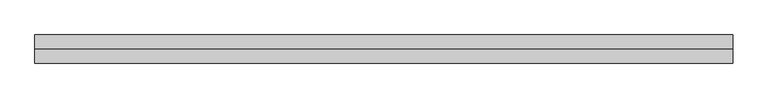
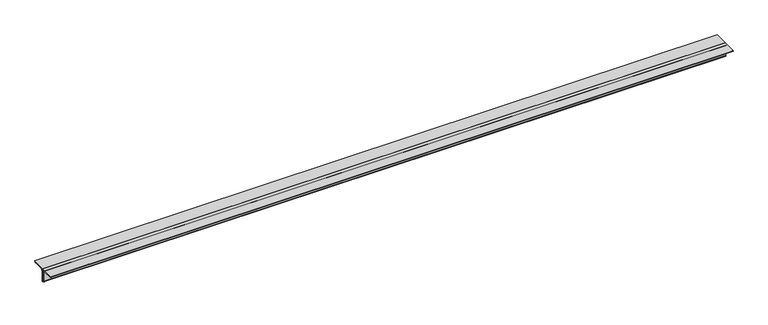
"""IFC4 building model written with IfcOpenShell, lengths in millimetres: member geometry, Steel Framing_2Ls_KS : H_SB_AR_S02_2Ls-100x100x10_VBR1."""

from ifc_helpers import new_model, si_unit, point, frame, frame_2d, origin, place, context, project, spatial, polyline, circle_curve, trimmed, segment, composite_curve, outline, extrude, source, transform, mapped, element, save


def member_093f2165(model_context):
    return source(origin(), model_context, "Body", "SweptSolid", [
        extrude(outline(composite_curve([segment(polyline([(0.0, 28.2), (100.0, 28.2)]), True, "CONTINUOUS"), segment(trimmed(circle_curve(frame_2d((90.0, 28.2)), 10.0), [point((100.0, 28.2))], [point((90.0, 18.2))], False, "CARTESIAN"), True, "CONTINUOUS"), segment(polyline([(90.0, 18.2), (20.0, 18.2)]), True, "CONTINUOUS"), segment(trimmed(circle_curve(frame_2d((20.0, 8.2)), 10.0), [point((20.0, 18.2))], [point((10.0, 8.2))], True, "CARTESIAN"), True, "CONTINUOUS"), segment(polyline([(10.0, 8.2), (10.0, -61.8)]), True, "CONTINUOUS"), segment(trimmed(circle_curve(frame_2d((0.0, -61.8)), 10.0), [point((10.0, -61.8))], [point((0.0, -71.8))], False, "CARTESIAN"), True, "CONTINUOUS"), segment(polyline([(0.0, -71.8), (0.0, 28.2)]), True, "CONTINUOUS")], self_intersect=False)), frame((-2479.1576866, 0.0, 0.0), z_axis=(1.0, 0.0, 0.0), x_axis=(0.0, 1.0, 0.0)), (0.0, 0.0, 1.0), 4958.3153733),
        extrude(outline(composite_curve([segment(polyline([(0.0, 28.2), (0.0, -71.8)]), True, "CONTINUOUS"), segment(trimmed(circle_curve(frame_2d((0.0, -61.8)), 10.0), [point((0.0, -71.8))], [point((-10.0, -61.8))], False, "CARTESIAN"), True, "CONTINUOUS"), segment(polyline([(-10.0, -61.8), (-10.0, 8.2)]), True, "CONTINUOUS"), segment(trimmed(circle_curve(frame_2d((-20.0, 8.2)), 10.0), [point((-10.0, 8.2))], [point((-20.0, 18.2))], True, "CARTESIAN"), True, "CONTINUOUS"), segment(polyline([(-20.0, 18.2), (-90.0, 18.2)]), True, "CONTINUOUS"), segment(trimmed(circle_curve(frame_2d((-90.0, 28.2)), 10.0), [point((-90.0, 18.2))], [point((-100.0, 28.2))], False, "CARTESIAN"), True, "CONTINUOUS"), segment(polyline([(-100.0, 28.2), (0.0, 28.2)]), True, "CONTINUOUS")], self_intersect=False)), frame((-2479.1576866, 0.0, 0.0), z_axis=(1.0, 0.0, 0.0), x_axis=(0.0, 1.0, 0.0)), (0.0, 0.0, 1.0), 4958.3153733),
    ])


if __name__ == "__main__":
    model = new_model("IFC4")
    model_context = context("Model", 3, world=origin())
    ifc_project = project(units=[si_unit("LENGTHUNIT", "METRE", prefix="MILLI")], contexts=[model_context])
    site = spatial("IfcSite", under=ifc_project)
    building = spatial("IfcBuilding", under=site)
    placement = place(None, origin())
    member_shape = member_093f2165(model_context)
    element("IfcMember", 1, ObjectType="Steel Framing_2Ls_KS : H_SB_AR_S02_2Ls-100x100x10_VBR1", at=placement, inside=building, context=model_context, shape_type="MappedRepresentation", body=[
        mapped(member_shape, transform((0.0, 0.0, 0.0), x_axis=(1.0, 0.0, 0.0), y_axis=(0.0, 1.0, 0.0), z_axis=(0.0, 0.0, 1.0))),
    ])
    save(model, "model.ifc")

# Revit data of these elements
# Type "Steel Framing_2Ls_KS : H_SB_AR_S02_2Ls-100x100x10_VBR1"
#   Type Comments = "MAIN"
#   Type Mark = "VBR1"
#   H_SectionID = "2Ls-100x100x10"
#   Assembly Code = "B10"
#   Legs = "LLBB"
#   H_Ratio for Additional Steel Plate = 0.2
#   W = 0
#   Perimeter = 0.80 m²/m
#   Nominal Weight = 29.80 kgf/m
#   Length [instance default] = 1524 mm
#   Space = 0 mm
#   b = 100 mm
#   d = 100 mm
#   t = 10 mm
#   y = 28.2 mm
#   A = 0.0038 m²
#   Structural Material [instance default] = Steel, 45-345
# Element 1 (IfcMember, "Steel Framing_2Ls_KS : H_SB_AR_S02_2Ls-100x100x10_VBR1")
#   Materials on its faces: "Steel, 45-345"
# Materials
#   "Steel, 45-345": class "Metal", colour RGB 189 187 185, transparency 0, Description = "Steel 345 MPa", Cost = 0
